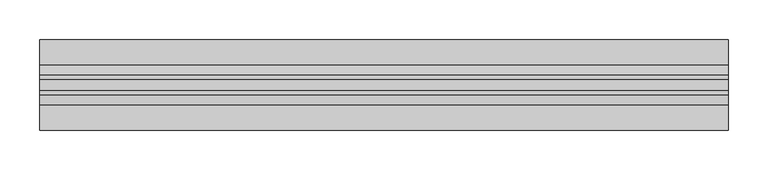
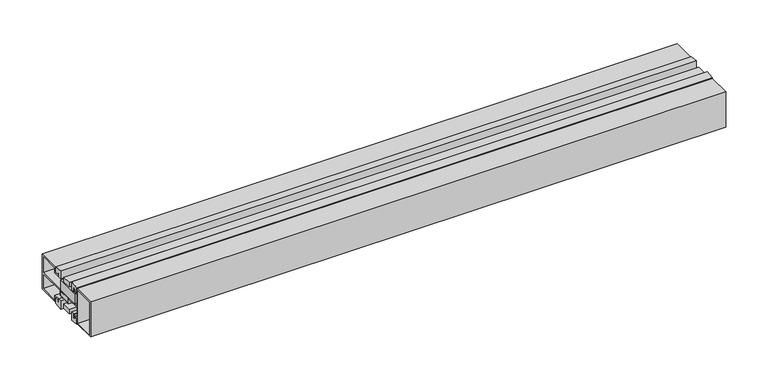
"""IFC4 building model written with IfcOpenShell, lengths in millimetres: proxy geometry, Generic Models 3:Generic Models 1:3:Generic Models 1:3 : Generic Models 3:Generic Models 1:300625:336034:Generic Models 1:3:Generic Models 1:3 : Generic Models 3:Generic Models 1:300625:336034 : Generic Models 3:Generic Models 1:3:Generic Models 1:3 : Generic Models 3:Generic Models 1:300625:336034:1 : Generic Models 3:Generic Models 1:3:Generic Models 1:3 : Generic Models 3:Generic Models 1:300625:336034:Generic Models 1:3:Generic Models 1:3 : Generic Models 3:Generic Models 1:300625:336034 : Generic Models 3:Generic Models 1:3:Generic Models 1:3 : Generic Models 3:Generic Models 1:300625:336034:301191."""

from ifc_helpers import new_model, si_unit, frame, origin, place, context, project, spatial, polyline, outline, extrude, source, transform, mapped, element, save


def generic_models_f1c34fde(model_context):
    return source(origin(), model_context, "Body", "SweptSolid", [
        extrude(outline(polyline([(593680.9367239, -579054.6832724), (593680.9367239, -579067.3832724), (592812.5742239, -579067.3832724), (592812.5742239, -579054.6832724), (593680.9367239, -579054.6832724)])), frame((0.0, 0.0, 2441.2521298), z_axis=(0.0, 0.0, 1.0), x_axis=(1.0, 0.0, 0.0)), (0.0, 0.0, 1.0), 6.3435484),
        extrude(outline(polyline([(-579086.0195091, 2437.3831629), (-579086.0195091, 2445.2228723), (-579081.7214373, 2445.2228723), (-579081.7214373, 2442.2790126), (-579078.8757591, 2442.2790126), (-579078.8757591, 2447.9925532), (-579074.1217032, 2447.9925532), (-579074.1217032, 2435.9222961), (-579086.0195091, 2437.3831629)])), frame((592812.5742239, 0.0, 0.0), z_axis=(1.0, 0.0, 0.0), x_axis=(0.0, 1.0, 0.0)), (0.0, 0.0, 1.0), 868.3625),
        extrude(outline(polyline([(-579043.1907857, 2442.2790126), (-579040.3451075, 2442.2790126), (-579040.3451075, 2445.2228723), (-579036.0470357, 2445.2228723), (-579036.0470357, 2437.3831629), (-579047.9448415, 2435.9222961), (-579047.9448415, 2447.9925532), (-579043.1907857, 2447.9925532), (-579043.1907857, 2442.2790126)])), frame((592812.5742239, 0.0, 0.0), z_axis=(1.0, 0.0, 0.0), x_axis=(0.0, 1.0, 0.0)), (0.0, 0.0, 1.0), 868.3625),
        extrude(outline(polyline([(593680.9367239, -579047.2017564), (593680.9367239, -579080.4885915), (592812.5742239, -579080.4885915), (592812.5742239, -579047.2017564), (593680.9367239, -579047.2017564)])), frame((0.0, 0.0, 2463.7831117), z_axis=(0.0, 0.0, 1.0), x_axis=(1.0, 0.0, 0.0)), (0.0, 0.0, 1.0), 14.2115027),
        extrude(outline(polyline([(593680.9367239, -579047.8857325), (593680.9367239, -579063.9971687), (592812.5742239, -579063.9971687), (592812.5742239, -579047.8857325), (593680.9367239, -579047.8857325)])), frame((0.0, 0.0, 2455.803391), z_axis=(0.0, 0.0, 1.0), x_axis=(1.0, 0.0, 0.0)), (0.0, 0.0, 1.0), 6.0797872),
        extrude(outline(polyline([(593680.9367239, -579054.6832724), (593680.9367239, -579067.3832724), (592812.5742239, -579067.3832724), (592812.5742239, -579054.6832724), (593680.9367239, -579054.6832724)])), frame((0.0, 0.0, 2479.9705452), z_axis=(0.0, 0.0, 1.0), x_axis=(1.0, 0.0, 0.0)), (0.0, 0.0, 1.0), 6.3435484),
        extrude(outline(polyline([(-579078.8757591, 2485.2872108), (-579081.7214373, 2485.2872108), (-579081.7214373, 2482.3433511), (-579086.0195091, 2482.3433511), (-579086.0195091, 2490.1830605), (-579074.1217032, 2491.6439273), (-579074.1217032, 2479.5736702), (-579078.8757591, 2479.5736702), (-579078.8757591, 2485.2872108)])), frame((592812.5742239, 0.0, 0.0), z_axis=(1.0, 0.0, 0.0), x_axis=(0.0, 1.0, 0.0)), (0.0, 0.0, 1.0), 868.3625),
        extrude(outline(polyline([(-579036.0470357, 2490.1830605), (-579036.0470357, 2482.3433511), (-579040.3451075, 2482.3433511), (-579040.3451075, 2485.2872108), (-579043.1907857, 2485.2872108), (-579043.1907857, 2479.5736702), (-579047.9448415, 2479.5736702), (-579047.9448415, 2491.6439273), (-579036.0470357, 2490.1830605)])), frame((592812.5742239, 0.0, 0.0), z_axis=(1.0, 0.0, 0.0), x_axis=(0.0, 1.0, 0.0)), (0.0, 0.0, 1.0), 868.3625),
        extrude(outline(polyline([(-579118.1663841, 2438.4), (-579118.1663841, 2489.1662234), (-579086.4163841, 2489.1662234), (-579086.4163841, 2481.9464761), (-579081.3245623, 2481.9464761), (-579081.3245623, 2484.8903358), (-579079.2726341, 2484.8903358), (-579079.2726341, 2479.9705452), (-579086.4163841, 2479.9705452), (-579086.4163841, 2463.7831117), (-579059.1333389, 2463.7831117), (-579059.1333389, 2461.8831782), (-579063.9971687, 2461.8831782), (-579063.9971687, 2455.803391), (-579059.1333389, 2455.803391), (-579059.1333389, 2454.5114362), (-579065.8971022, 2454.5114362), (-579065.8971022, 2461.8831782), (-579086.4163841, 2461.8831782), (-579086.4163841, 2447.6716755), (-579079.2726341, 2447.6716755), (-579079.2726341, 2443.1005159), (-579081.3245623, 2443.1005159), (-579081.3245623, 2445.6197473), (-579086.4163841, 2445.6197473), (-579086.4163841, 2438.4), (-579118.1663841, 2438.4)]), holes=[polyline([(-579088.3163176, 2487.2662899), (-579115.6584719, 2487.2662899), (-579115.6584719, 2440.2999335), (-579088.3163176, 2440.2999335), (-579088.3163176, 2487.2662899)])]), frame((592812.5742239, 0.0, 0.0), z_axis=(1.0, 0.0, 0.0), x_axis=(0.0, 1.0, 0.0)), (0.0, 0.0, 1.0), 868.3625),
        extrude(outline(polyline([(-579040.7419825, 2484.8903358), (-579040.7419825, 2481.9464761), (-579035.6501607, 2481.9464761), (-579035.6501607, 2489.1662234), (-579003.8663841, 2489.1662234), (-579003.8663841, 2438.4), (-579035.6501607, 2438.4), (-579035.6501607, 2445.6197473), (-579040.7419825, 2445.6197473), (-579040.7419825, 2443.1005159), (-579042.7939107, 2443.1005159), (-579042.7939107, 2447.6716755), (-579033.7502272, 2447.6716755), (-579033.7502272, 2440.3222126), (-579005.8423149, 2440.3222126), (-579005.8423149, 2461.8831782), (-579045.985799, 2461.8831782), (-579045.985799, 2454.5114362), (-579052.7495623, 2454.5114362), (-579052.7495623, 2455.803391), (-579047.8857325, 2455.803391), (-579047.8857325, 2461.8831782), (-579052.7495623, 2461.8831782), (-579052.7495623, 2463.7831117), (-579005.8423149, 2463.7831117), (-579005.8423149, 2487.2564243), (-579033.7502272, 2487.2564243), (-579033.7502272, 2479.9705452), (-579042.7939107, 2479.9705452), (-579042.7939107, 2484.8903358), (-579040.7419825, 2484.8903358)])), frame((592812.5742239, 0.0, 0.0), z_axis=(1.0, 0.0, 0.0), x_axis=(0.0, 1.0, 0.0)), (0.0, 0.0, 1.0), 868.3625),
    ])


if __name__ == "__main__":
    model = new_model("IFC4")
    model_context = context("Model", 3, world=origin())
    ifc_project = project(units=[si_unit("LENGTHUNIT", "METRE", prefix="MILLI")], contexts=[model_context])
    site = spatial("IfcSite", under=ifc_project)
    building = spatial("IfcBuilding", under=site)
    placement = place(None, origin())
    generic_models_shape = generic_models_f1c34fde(model_context)
    element("IfcBuildingElementProxy", 1, Name="Generic Models 3:Generic Models 1:3:Generic Models 1:3 : Generic Models 3:Generic Models 1:300625:336034:Generic Models 1:3:Generic Models 1:3 : Generic Models 3:Generic Models 1:300625:336034 : Generic Models 3:Generic Models 1:3:Generic Models 1:3 : Generic Models 3:Generic Models 1:300625:336034:1 : Generic Models 3:Generic Models 1:3:Generic Models 1:3 : Generic Models 3:Generic Models 1:300625:336034:Generic Models 1:3:Generic Models 1:3 : Generic Models 3:Generic Models 1:300625:336034 : Generic Models 3:Generic Models 1:3:Generic Models 1:3 : Generic Models 3:Generic Models 1:300625:336034:301191", ObjectType="Generic Models 3:Generic Models 1:3:Generic Models 1:3 : Generic Models 3:Generic Models 1:300625:336034:Generic Models 1:3:Generic Models 1:3 : Generic Models 3:Generic Models 1:300625:336034 : Generic Models 3:Generic Models 1:3:Generic Models 1:3 : Generic Models 3:Generic Models 1:300625:336034:1 : Generic Models 3:Generic Models 1:3:Generic Models 1:3 : Generic Models 3:Generic Models 1:300625:336034:Generic Models 1:3:Generic Models 1:3 : Generic Models 3:Generic Models 1:300625:336034 : Generic Models 3:Generic Models 1:3:Generic Models 1:3 : Generic Models 3:Generic Models 1:300625:336034:301191", at=placement, inside=building, context=model_context, shape_type="MappedRepresentation", body=[
        mapped(generic_models_shape, transform((0.0, 0.0, 0.0), x_axis=(1.0, 0.0, 0.0), y_axis=(0.0, 1.0, 0.0), z_axis=(0.0, 0.0, 1.0))),
    ])
    save(model, "model.ifc")

# Revit data of these elements
# Type "Generic Models 3:Generic Models 1:3:Generic Models 1:3 : Generic Models 3:Generic Models 1:300625:336034:Generic Models 1:3:Generic Models 1:3 : Generic Models 3:Generic Models 1:300625:336034 : Generic Models 3:Generic Models 1:3:Generic Models 1:3 : Generic Models 3:Generic Models 1:300625:336034:1 : Generic Models 3:Generic Models 1:3:Generic Models 1:3 : Generic Models 3:Generic Models 1:300625:336034:Generic Models 1:3:Generic Models 1:3 : Generic Models 3:Generic Models 1:300625:336034 : Generic Models 3:Generic Models 1:3:Generic Models 1:3 : Generic Models 3:Generic Models 1:300625:336034:301191"
#   NameOverride = "Generic Models 3:Generic Models 1:3:Generic Models 1:3 : Generic Models 3:Generic Models 1:300625:336034:Generic Models 1:3:Generic Models 1:3 : Generic Models 3:Generic Models 1:300625:336034 : Generic Models 3:Generic Models 1:3:Generic Models 1:3 : Generic Models 3:Generic Models 1:300625:336034:301191"
#   ObjectTypeOverride = "Generic Models 1:3:Generic Models 1:3 : Generic Models 3:Generic Models 1:300625:336034 : Generic Models 3:Generic Models 1:3:Generic Models 1:3 : Generic Models 3:Generic Models 1:300625:336034"
#   Reference = "Generic Models 1"
#   Tag = "301191"
# Element 1 (IfcBuildingElementProxy, "Generic Models 3:Generic Models 1:3:Generic Models 1:3 : Generic Models 3:Generic Models 1:300625:336034:Generic Models 1:3:Generic Models 1:3 : Generic Models 3:Generic Models 1:300625:336034 : Generic Models 3:Generic Models 1:3:Generic Models 1:3 : Generic Models 3:Generic Models 1:300625:336034:1 : Generic Models 3:Generic Models 1:3:Generic Models 1:3 : Generic Models 3:Generic Models 1:300625:336034:Generic Models 1:3:Generic Models 1:3 : Generic Models 3:Generic Models 1:300625:336034 : Generic Models 3:Generic Models 1:3:Generic Models 1:3 : Generic Models 3:Generic Models 1:300625:336034:301191")
#   Materials on its faces: "THERMAL BROKEN ALUMINUM STOREFRONT"
# Materials
#   "THERMAL BROKEN ALUMINUM STOREFRONT": class "Unassigned", colour RGB 244 244 244, transparency 0, Cost = 0
